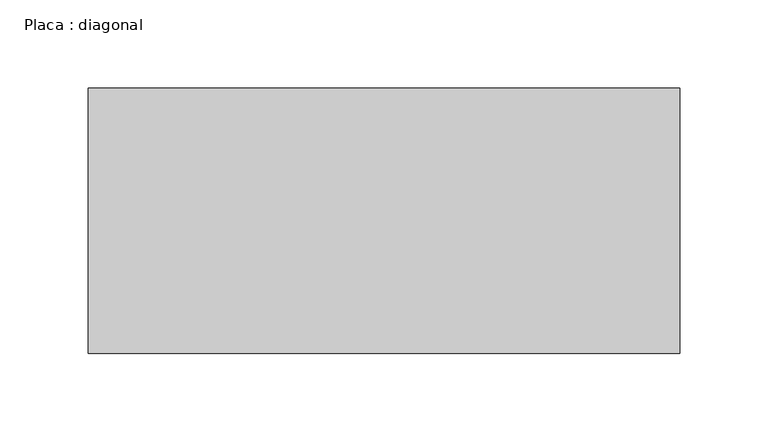
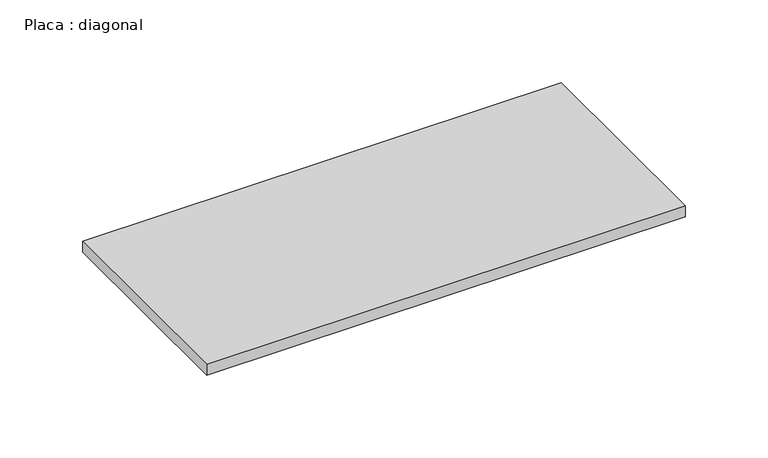
"""IFC4 building model written with IfcOpenShell, lengths in millimetres: beam geometry, Placa : diagonal."""

from ifc_helpers import new_model, si_unit, frame, origin, place, context, project, spatial, polyline, outline, extrude, source, transform, mapped, element, save


def placa_diagonal_7fe59f73(model_context):
    return source(origin(), model_context, "Body", "SweptSolid", [
        extrude(outline(polyline([(166.951958, 75.0), (166.951958, -75.0), (-167.3065458, -75.0), (-167.3065458, 75.0), (166.951958, 75.0)])), frame((0.0, 0.0, -4.0), z_axis=(0.0, 0.0, 1.0), x_axis=(1.0, 0.0, 0.0)), (0.0, 0.0, 1.0), 8.0),
    ])


if __name__ == "__main__":
    model = new_model("IFC4")
    model_context = context("Model", 3, world=origin())
    ifc_project = project(units=[si_unit("LENGTHUNIT", "METRE", prefix="MILLI")], contexts=[model_context])
    site = spatial("IfcSite", under=ifc_project)
    building = spatial("IfcBuilding", under=site)
    placement = place(None, origin())
    placa_diagonal_shape = placa_diagonal_7fe59f73(model_context)
    element("IfcBeam", 1, ObjectType="Placa : diagonal", at=placement, inside=building, context=model_context, shape_type="MappedRepresentation", body=[
        mapped(placa_diagonal_shape, transform((0.0, 0.0, 0.0), x_axis=(1.0, 0.0, 0.0), y_axis=(0.0, 1.0, 0.0), z_axis=(0.0, 0.0, 1.0))),
    ])
    save(model, "model.ifc")

# Revit data of these elements
# Type "Placa : diagonal"
#   W = 0
#   Length [instance default] = 1.50 m
#   b = 0.15 m
#   d = 0.008 m
#   A = 0 m²
#   Structural Material [instance default] = Aço, 45-345
# Element 1 (IfcBeam, "Placa : diagonal")
#   Materials on its faces: "Aço, 45-345"
# Materials
#   "Aço, 45-345": class "Metal", colour RGB 247 247 247, transparency 0, Description = "Aço 345 MPa", Cost = 0
